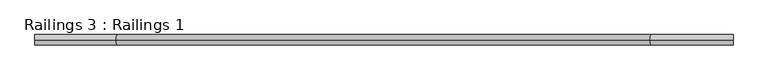
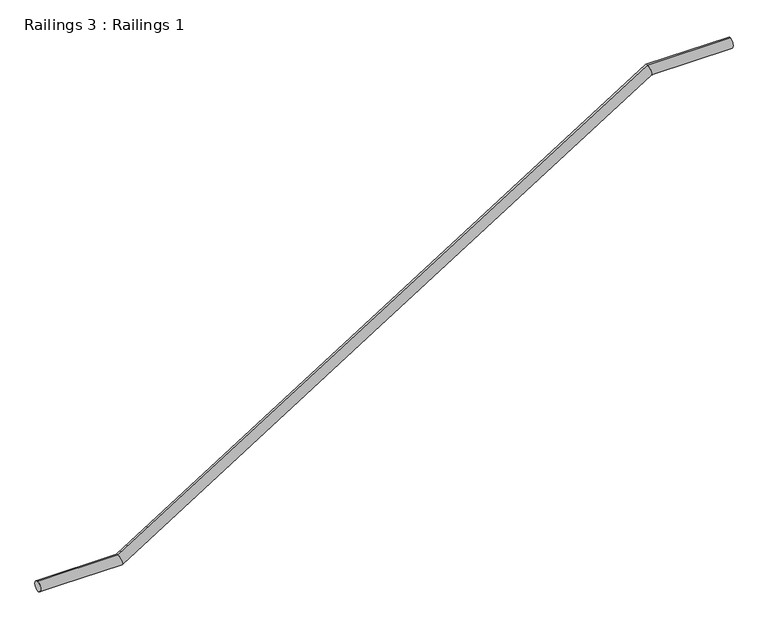
"""IFC4 building model written with IfcOpenShell, lengths in millimetres: railing geometry, Railings 3 : Railings 1."""

from ifc_helpers import new_model, si_unit, frame, origin, place, context, project, spatial, circle_curve, ellipse_curve, source, transform, mapped, element, save
from ifc_brep_helpers import plane_surface, cylinder_surface, advanced_brep


def railings_3_railings_1_a42c2f52(model_context):
    return source(origin(), model_context, "Body", "AdvancedBrep", [
        advanced_brep(
        [(24461.7840778, 25902.7078032, 268856.61875), (24461.7840778, 25902.7078032, 268818.51875), (27052.5840778, 25902.7078032, 270100.4971591), (27052.5840778, 25902.7078032, 270062.3971591), (24761.0995713, 25902.7078032, 268856.61875), (24772.0685843, 25902.7078032, 268818.51875), (26742.2995713, 25902.7078032, 270100.4971591), (26753.2685843, 25902.7078032, 270062.3971591)],
        [
            (0, 1, circle_curve(frame((24461.7840778, 25902.7078032, 268837.56875), z_axis=(-1.0, 0.0, 0.0), x_axis=(0.0, 0.0, -1.0)), 19.05)),
            (1, 0, circle_curve(frame((24461.7840778, 25902.7078032, 268837.56875), z_axis=(-1.0, 0.0, 0.0), x_axis=(0.0, 0.0, -1.0)), 19.05)),
            (2, 3, circle_curve(frame((27052.5840778, 25902.7078032, 270081.4471591), z_axis=(1.0, 0.0, 0.0), x_axis=(0.0, 0.0, -1.0)), 19.05)),
            (3, 2, circle_curve(frame((27052.5840778, 25902.7078032, 270081.4471591), z_axis=(1.0, 0.0, 0.0), x_axis=(0.0, 0.0, -1.0)), 19.05)),
            (0, 4),
            (4, 5, ellipse_curve(frame((24766.5840778, 25902.7078032, 268837.56875), z_axis=(-0.9609670094755167, 0.0, -0.2766629839708993), x_axis=(-0.27666298397089967, 0.0, 0.9609670094755168)), 19.8237815, 19.05)),
            (5, 1),
            (5, 4, ellipse_curve(frame((24766.5840778, 25902.7078032, 268837.56875), z_axis=(-0.9609670094755167, 0.0, -0.2766629839708993), x_axis=(-0.27666298397089967, 0.0, 0.9609670094755168)), 19.8237815, 19.05)),
            (4, 6),
            (6, 7, ellipse_curve(frame((26747.7840778, 25902.7078032, 270081.4471591), z_axis=(-0.9609670094755167, 0.0, -0.2766629839708993), x_axis=(0.27666298397089895, 0.0, -0.9609670094755169)), 19.8237815, 19.05)),
            (7, 5),
            (7, 6, ellipse_curve(frame((26747.7840778, 25902.7078032, 270081.4471591), z_axis=(-0.9609670094755167, 0.0, -0.2766629839708993), x_axis=(0.27666298397089895, 0.0, -0.9609670094755169)), 19.8237815, 19.05)),
            (6, 2),
            (3, 7),
        ],
        [
            plane_surface(frame((24461.7840778, 25883.6578032, 268837.56875), z_axis=(-1.0, 0.0, 0.0), x_axis=(0.0, -1.0, 0.0))),
            plane_surface(frame((27052.5840778, 25883.6578032, 270081.4471591), z_axis=(1.0, 0.0, 0.0), x_axis=(0.0, -1.0, 0.0))),
            cylinder_surface(frame((24461.7840778, 25902.7078032, 268837.56875), z_axis=(-1.0, 0.0, 0.0), x_axis=(0.0, 0.0, -1.0)), 19.05),
            cylinder_surface(frame((24766.5840778, 25902.7078032, 268837.56875), z_axis=(-0.8469151866006359, 0.0, -0.5317280006781757), x_axis=(0.5317280006781757, 0.0, -0.8469151866006359)), 19.05),
            cylinder_surface(frame((26747.7840778, 25902.7078032, 270081.4471591), z_axis=(-1.0, 0.0, 0.0), x_axis=(0.0, 0.0, -1.0)), 19.05),
        ],
        [
            (0, [[1, 2]]),
            (1, [[3, 4]]),
            (2, [[-1, 5, 6, 7]]),
            (2, [[-2, -7, 8, -5]]),
            (3, [[-6, 9, 10, 11]]),
            (3, [[-8, -11, 12, -9]]),
            (4, [[-10, 13, -4, 14]]),
            (4, [[-12, -14, -3, -13]]),
        ],
    ),
    ])


if __name__ == "__main__":
    model = new_model("IFC4")
    model_context = context("Model", 3, world=origin())
    ifc_project = project(units=[si_unit("LENGTHUNIT", "METRE", prefix="MILLI")], contexts=[model_context])
    site = spatial("IfcSite", under=ifc_project)
    building = spatial("IfcBuilding", under=site)
    placement = place(None, origin())
    railings_3_railings_1_shape = railings_3_railings_1_a42c2f52(model_context)
    element("IfcRailing", 1, ObjectType="Railings 3 : Railings 1", at=placement, inside=building, context=model_context, shape_type="MappedRepresentation", body=[
        mapped(railings_3_railings_1_shape, transform((0.0, 0.0, 0.0), x_axis=(1.0, 0.0, 0.0), y_axis=(0.0, 1.0, 0.0), z_axis=(0.0, 0.0, 1.0))),
    ])
    save(model, "model.ifc")

# Revit data of these elements
# Element 1 (IfcRailing, "Railings 3 : Railings 1")
#   Materials on its faces: "ALUM. RAILING"
# Materials
#   "ALUM. RAILING": class "Generic", colour RGB 255 255 255, transparency 0, Cost = 0
